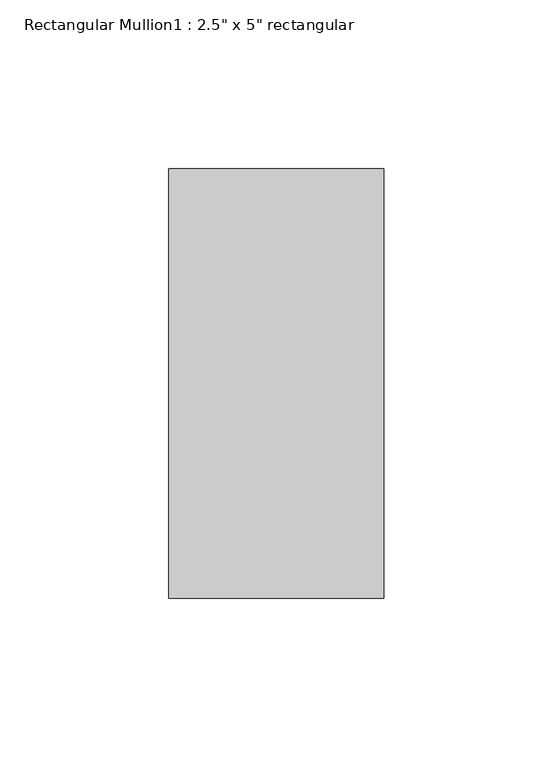
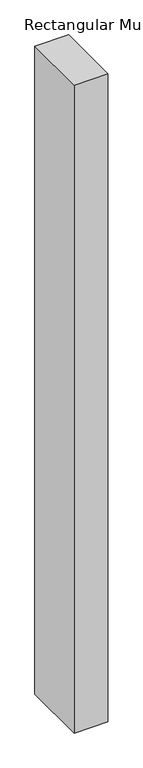
"""IFC4 building model written with IfcOpenShell, lengths in millimetres: member geometry."""

import ifcopenshell
import ifcopenshell.guid

model = None  # the IFC model being written
_history = None  # IfcOwnerHistory: only IFC2X3 demands one
_inside = {}  # id of a spatial element -> (the spatial element, [elements in it])
_under = {}  # id of a project, library or spatial element -> (it, [spatial elements below it])
_declared = {}  # id of a project -> (the project, [libraries it declares])
_typed = {}  # id of a type object -> (the type object, [elements of that type])
_made_of = {}  # id of a material, layer set ... -> (it, [elements and type objects made of it])


def new_model(schema):
    """Start an empty IFC model of exactly this schema.

    Asked for "IFC4X3", IfcOpenShell would pick the latest addendum, in which some entities
    have other attributes; the version numbers below select the first issue.
    IFC2X3 requires an IfcOwnerHistory on every rooted entity: one is made here for all.
    """
    global model, _history
    if schema == "IFC4X3":
        model = ifcopenshell.file(schema_version=(4, 3, 0, 0))
    else:
        model = ifcopenshell.file(schema=schema)
    _inside.clear()
    _under.clear()
    _declared.clear()
    _typed.clear()
    _made_of.clear()
    _history = None
    if model.schema == "IFC2X3":
        org = make("IfcOrganization", Name="unknown")
        user = make(
            "IfcPersonAndOrganization",
            ThePerson=make("IfcPerson", FamilyName="unknown"),
            TheOrganization=org,
        )
        app = make(
            "IfcApplication",
            ApplicationDeveloper=org,
            Version="unknown",
            ApplicationFullName="unknown",
            ApplicationIdentifier="unknown",
        )
        _history = make(
            "IfcOwnerHistory",
            OwningUser=user,
            OwningApplication=app,
            ChangeAction="ADDED",
            CreationDate=0,
        )
    return model


def make(cls, **values):
    """One entity of the class cls with the attributes given. An attribute that is None is left unset."""
    return model.create_entity(
        cls, **{name: value for name, value in values.items() if value is not None}
    )


def rooted(cls, **values):
    """An entity with a GlobalId (a new one), such as an element, a storey or a relation."""
    return make(cls, GlobalId=ifcopenshell.guid.new(), OwnerHistory=_history, **values)


def si_unit(unit_type, name, prefix=None):
    """IfcSIUnit, for example si_unit("LENGTHUNIT", "METRE", prefix="MILLI")."""
    return make("IfcSIUnit", UnitType=unit_type, Prefix=prefix, Name=name)


def assignment(units):
    """IfcUnitAssignment: the units of a project."""
    return None if units is None else make("IfcUnitAssignment", Units=units)


def point(xyz):
    """IfcCartesianPoint."""
    return None if xyz is None else make("IfcCartesianPoint", Coordinates=xyz)


def direction(xyz):
    """IfcDirection."""
    return None if xyz is None else make("IfcDirection", DirectionRatios=xyz)


def frame(location, z_axis=None, x_axis=None):
    """IfcAxis2Placement3D, a coordinate frame: its origin and axes. An axis left out is left unset."""
    return make(
        "IfcAxis2Placement3D",
        Location=point(location),
        Axis=direction(z_axis),
        RefDirection=direction(x_axis),
    )


def origin():
    """The frame at (0, 0, 0) with its axes left unset."""
    return frame((0.0, 0.0, 0.0))


def place(relative_to, where):
    """IfcLocalPlacement: puts the frame where relative to a parent placement (None: the world)."""
    return make(
        "IfcLocalPlacement", PlacementRelTo=relative_to, RelativePlacement=where
    )


def context(
    kind, dimensions, precision=None, world=None, true_north=None, identifier=None
):
    """IfcGeometricRepresentationContext, for example the 3D "Model" context."""
    return make(
        "IfcGeometricRepresentationContext",
        ContextIdentifier=identifier,
        ContextType=kind,
        CoordinateSpaceDimension=dimensions,
        Precision=precision,
        WorldCoordinateSystem=world,
        TrueNorth=true_north,
    )


def project(units=None, contexts=None):
    """IfcProject with its units and contexts."""
    return rooted(
        "IfcProject",
        Name="project",
        RepresentationContexts=contexts,
        UnitsInContext=assignment(units),
    )


def spatial(cls, under=None, at=None, **own):
    """A site, building, storey or space (cls), placed at a placement, below another one or the project."""
    s = rooted(cls, ObjectPlacement=at, **own)
    if under is not None:
        _under.setdefault(under.id(), (under, []))[1].append(s)
    return s


def polyline(points):
    """IfcPolyline through the points."""
    return make("IfcPolyline", Points=[point(p) for p in points])


def outline(outer, holes=None, kind="AREA"):
    """IfcArbitraryClosedProfileDef: a profile drawn as a closed curve; with holes, ...WithVoids."""
    if holes is None:
        return make("IfcArbitraryClosedProfileDef", ProfileType=kind, OuterCurve=outer)
    return make(
        "IfcArbitraryProfileDefWithVoids",
        ProfileType=kind,
        OuterCurve=outer,
        InnerCurves=holes,
    )


def extrude(swept, where, along, depth):
    """IfcExtrudedAreaSolid: the profile swept, set in the frame where, extruded along a direction by depth."""
    return make(
        "IfcExtrudedAreaSolid",
        SweptArea=swept,
        Position=where,
        ExtrudedDirection=direction(along),
        Depth=depth,
    )


def shape(context_of_items, identifier, shape_type, items):
    """IfcShapeRepresentation: the items that make up one representation, for example the "Body"."""
    return make(
        "IfcShapeRepresentation",
        ContextOfItems=context_of_items,
        RepresentationIdentifier=identifier,
        RepresentationType=shape_type,
        Items=items,
    )


def source(mapping_origin, context_of_items, identifier, shape_type, items):
    """IfcRepresentationMap: a shape defined once, which mapped items show again and again."""
    return make(
        "IfcRepresentationMap",
        MappingOrigin=mapping_origin,
        MappedRepresentation=shape(context_of_items, identifier, shape_type, items),
    )


def transform(
    local_origin,
    x_axis=None,
    y_axis=None,
    z_axis=None,
    scale=None,
    scale2=None,
    scale3=None,
    uniform=True,
):
    """IfcCartesianTransformationOperator3D, or its non-uniform kind. x_axis, y_axis, z_axis: its Axis1, 2, 3."""
    if uniform:
        return make(
            "IfcCartesianTransformationOperator3D",
            Axis1=direction(x_axis),
            Axis2=direction(y_axis),
            LocalOrigin=point(local_origin),
            Scale=scale,
            Axis3=direction(z_axis),
        )
    return make(
        "IfcCartesianTransformationOperator3DnonUniform",
        Axis1=direction(x_axis),
        Axis2=direction(y_axis),
        LocalOrigin=point(local_origin),
        Scale=scale,
        Axis3=direction(z_axis),
        Scale2=scale2,
        Scale3=scale3,
    )


def mapped(mapping_source, mapping_target):
    """IfcMappedItem: shows the shape of a source again, moved by a transform."""
    return make(
        "IfcMappedItem", MappingSource=mapping_source, MappingTarget=mapping_target
    )


def made_of(thing, what):
    """Note that an element or type object is made of a material, layer set ...; save() writes the relation."""
    if what is not None:
        _made_of.setdefault(what.id(), (what, []))[1].append(thing)
    return thing


def element(
    cls,
    number,
    at=None,
    inside=None,
    cuts=None,
    type_object=None,
    material=None,
    context=None,
    identifier="Body",
    shape_type=None,
    held_by="IfcProductDefinitionShape",
    body=None,
    shapes=None,
    **own,
):
    """One element of the class cls, such as IfcWall. Its Tag is "e" and its number.

    at: its placement. inside: the storey or other place that contains it. cuts: it is an
    opening in that element (IfcRelVoidsElement). A single representation is given by context,
    identifier, shape_type and body (its items); several are given by shapes. held_by: the class
    of the entity that holds the representations. save() writes the other relations.
    """
    e = rooted(cls, Tag="e%d" % number, ObjectPlacement=at, **own)
    if body is not None:
        shapes = [shape(context, identifier, shape_type, body)]
    if shapes is not None:
        e.Representation = make(held_by, Representations=shapes)
    if inside is not None:
        _inside.setdefault(inside.id(), (inside, []))[1].append(e)
    if cuts is not None:
        rooted(
            "IfcRelVoidsElement", RelatingBuildingElement=cuts, RelatedOpeningElement=e
        )
    if type_object is not None:
        _typed.setdefault(type_object.id(), (type_object, []))[1].append(e)
    return made_of(e, material)


def aggregate(whole, parts):
    """IfcRelAggregates: a whole, such as a stair, and the parts it consists of."""
    return rooted("IfcRelAggregates", RelatingObject=whole, RelatedObjects=parts)


def save(model, path):
    """Write the relations noted so far, then the file.

    IfcRelAggregates (storeys below a building ...), IfcRelContainedInSpatialStructure (elements
    in a storey), IfcRelDefinesByType, IfcRelAssociatesMaterial and IfcRelDeclares: one each for
    every whole, place, type object, material and project.
    """
    for whole, parts in _under.values():
        aggregate(whole, parts)
    for where, things in _inside.values():
        rooted(
            "IfcRelContainedInSpatialStructure",
            RelatedElements=things,
            RelatingStructure=where,
        )
    for kind, things in _typed.values():
        rooted("IfcRelDefinesByType", RelatedObjects=things, RelatingType=kind)
    for what, things in _made_of.values():
        rooted("IfcRelAssociatesMaterial", RelatedObjects=things, RelatingMaterial=what)
    for by, libraries in _declared.values():
        rooted("IfcRelDeclares", RelatingContext=by, RelatedDefinitions=libraries)
    model.write(path)


def member_98b79ab6(model_context):
    return source(origin(), model_context, "Body", "SweptSolid", [
        extrude(outline(polyline([(31.75, 63.5), (31.75, -63.5), (-31.75, -63.5), (-31.75, 63.5), (31.75, 63.5)])), frame((0.0, 0.0, -1282.7), z_axis=(0.0, 0.0, 1.0), x_axis=(1.0, 0.0, 0.0)), (0.0, 0.0, 1.0), 1282.7),
    ])


if __name__ == "__main__":
    model = new_model("IFC4")
    model_context = context("Model", 3, world=origin())
    ifc_project = project(units=[si_unit("LENGTHUNIT", "METRE", prefix="MILLI")], contexts=[model_context])
    site = spatial("IfcSite", under=ifc_project)
    building = spatial("IfcBuilding", under=site)
    placement = place(None, origin())
    member_shape = member_98b79ab6(model_context)
    element("IfcMember", 1, ObjectType="Rectangular Mullion1 : 2.5\" x 5\" rectangular", at=placement, inside=building, context=model_context, shape_type="MappedRepresentation", body=[
        mapped(member_shape, transform((0.0, 0.0, 0.0), x_axis=(1.0, 0.0, 0.0), y_axis=(0.0, 1.0, 0.0), z_axis=(0.0, 0.0, 1.0))),
    ])
    save(model, "model.ifc")

# Revit data of these elements
# Type "Rectangular Mullion1 : 2.5\" x 5\" rectangular"
#   built-in parameter 1007304 = 0.416667 (stored number, unit not read)
#   built-in parameter 1007301 = 0.104167 (stored number, unit not read)
#   built-in parameter 1007300 = 0.104167 (stored number, unit not read)
# Element 1 (IfcMember, "Rectangular Mullion1 : 2.5\" x 5\" rectangular")
#   Materials on its faces: "support-frame"
# Materials
#   "support-frame": class "Unassigned", colour RGB 233 233 233, transparency 0, Cost = 0
